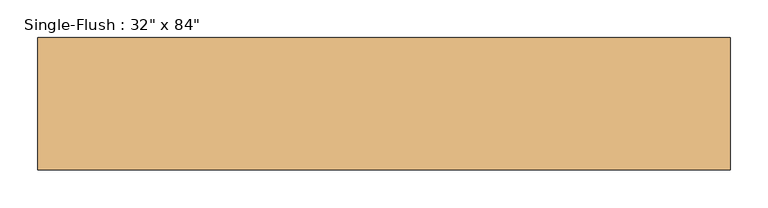
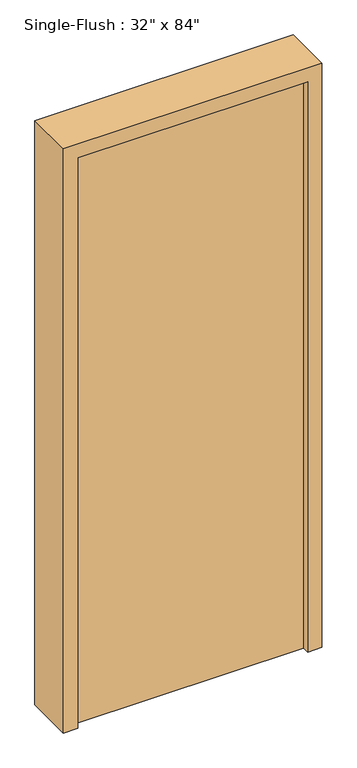
"""IFC4 building model written with IfcOpenShell, lengths in millimetres: door geometry."""

from ifc_helpers import new_model, si_unit, frame, origin, origin_with_axes, place, context, project, spatial, polyline, outline, extrude, source, transform, mapped, element, save


def door_7caa3a9d(model_context):
    return source(origin(), model_context, "Body", "SweptSolid", [
        extrude(outline(polyline([(2184.4, 457.2), (2184.4, -457.2), (0.0, -457.2), (0.0, -406.4), (2133.6, -406.4), (2133.6, 406.4), (0.0, 406.4), (0.0, 457.2), (2184.4, 457.2)])), frame((0.0, -87.3125, 0.0), z_axis=(0.0, 1.0, 0.0), x_axis=(0.0, 0.0, 1.0)), (0.0, 0.0, 1.0), 174.625),
        extrude(outline(polyline([(406.4, -11.1125), (406.4, -61.9125), (-406.4, -61.9125), (-406.4, -11.1125), (406.4, -11.1125)])), origin_with_axes(), (0.0, 0.0, 1.0), 2133.6),
    ])


if __name__ == "__main__":
    model = new_model("IFC4")
    model_context = context("Model", 3, world=origin())
    ifc_project = project(units=[si_unit("LENGTHUNIT", "METRE", prefix="MILLI")], contexts=[model_context])
    site = spatial("IfcSite", under=ifc_project)
    building = spatial("IfcBuilding", under=site)
    placement = place(None, origin())
    door_shape = door_7caa3a9d(model_context)
    element("IfcDoor", 1, ObjectType="Single-Flush : 32\" x 84\"", at=placement, inside=building, context=model_context, shape_type="MappedRepresentation", body=[
        mapped(door_shape, transform((0.0, 0.0, 0.0), x_axis=(1.0, 0.0, 0.0), y_axis=(0.0, 1.0, 0.0), z_axis=(0.0, 0.0, 1.0))),
    ])
    save(model, "model.ifc")

# Revit data of these elements
# Type "Single-Flush : 32\" x 84\""
#   Type Mark = "10"
#   Construction Type Id = "MDOOR"
#   Assembly Code = "C1020"
#   Analytic Construction = "Metal"
#   Thickness = 0' - 2"
#   Thermal Resistance (R) = 0.270117 (m²·K)/W
#   Heat Transfer Coefficient (U) = 3.7021 W/(m²·K)
#   Height = 7' - 0"
#   Trim Projection Ext = 0' - 1"
#   Trim Projection Int = 0' - 1"
#   Trim Width = 0' - 2"
#   Width = 2' - 8"
#   Door Material = Door - Panel
#   Frame Material = Door - Frame
#   Visual Light Transmittance = 0
#   Solar Heat Gain Coefficient = 0
#   Function = (empty or 0)
#   Wall Closure = (empty or 0)
# Element 1 (IfcDoor, "Single-Flush : 32\" x 84\"")
#   Materials on its faces: "Door - Frame", "Door - Panel"
# Materials
#   "Door - Panel": class "Wood", colour RGB 212 179 113, transparency 0, Cost = 0
#   "Door - Frame": class "Miscellaneous", colour RGB 65 65 65, transparency 0, Cost = 0
